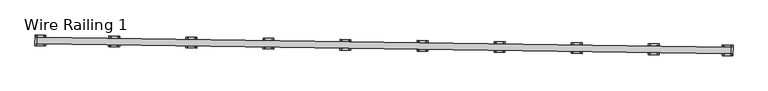
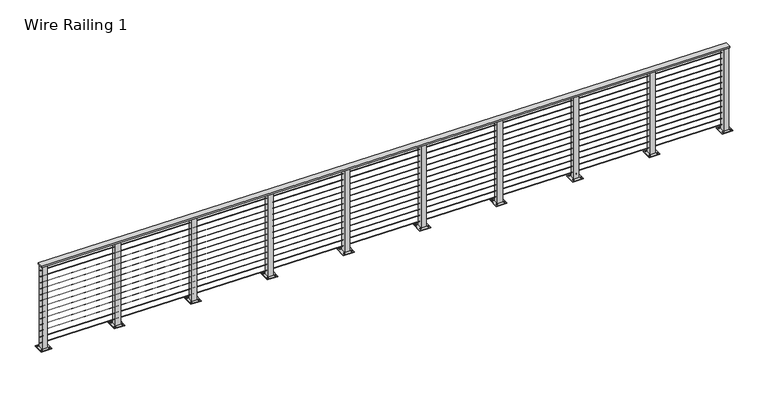
"""IFC4 building model written with IfcOpenShell, lengths in millimetres: railing geometry, Wire Railing 1."""

import ifcopenshell
import ifcopenshell.guid

model = None  # the IFC model being written
_history = None  # IfcOwnerHistory: only IFC2X3 demands one
_inside = {}  # id of a spatial element -> (the spatial element, [elements in it])
_under = {}  # id of a project, library or spatial element -> (it, [spatial elements below it])
_declared = {}  # id of a project -> (the project, [libraries it declares])
_typed = {}  # id of a type object -> (the type object, [elements of that type])
_made_of = {}  # id of a material, layer set ... -> (it, [elements and type objects made of it])


def new_model(schema):
    """Start an empty IFC model of exactly this schema.

    Asked for "IFC4X3", IfcOpenShell would pick the latest addendum, in which some entities
    have other attributes; the version numbers below select the first issue.
    IFC2X3 requires an IfcOwnerHistory on every rooted entity: one is made here for all.
    """
    global model, _history
    if schema == "IFC4X3":
        model = ifcopenshell.file(schema_version=(4, 3, 0, 0))
    else:
        model = ifcopenshell.file(schema=schema)
    _inside.clear()
    _under.clear()
    _declared.clear()
    _typed.clear()
    _made_of.clear()
    _history = None
    if model.schema == "IFC2X3":
        org = make("IfcOrganization", Name="unknown")
        user = make(
            "IfcPersonAndOrganization",
            ThePerson=make("IfcPerson", FamilyName="unknown"),
            TheOrganization=org,
        )
        app = make(
            "IfcApplication",
            ApplicationDeveloper=org,
            Version="unknown",
            ApplicationFullName="unknown",
            ApplicationIdentifier="unknown",
        )
        _history = make(
            "IfcOwnerHistory",
            OwningUser=user,
            OwningApplication=app,
            ChangeAction="ADDED",
            CreationDate=0,
        )
    return model


def make(cls, **values):
    """One entity of the class cls with the attributes given. An attribute that is None is left unset."""
    return model.create_entity(
        cls, **{name: value for name, value in values.items() if value is not None}
    )


def rooted(cls, **values):
    """An entity with a GlobalId (a new one), such as an element, a storey or a relation."""
    return make(cls, GlobalId=ifcopenshell.guid.new(), OwnerHistory=_history, **values)


def si_unit(unit_type, name, prefix=None):
    """IfcSIUnit, for example si_unit("LENGTHUNIT", "METRE", prefix="MILLI")."""
    return make("IfcSIUnit", UnitType=unit_type, Prefix=prefix, Name=name)


def assignment(units):
    """IfcUnitAssignment: the units of a project."""
    return None if units is None else make("IfcUnitAssignment", Units=units)


def point(xyz):
    """IfcCartesianPoint."""
    return None if xyz is None else make("IfcCartesianPoint", Coordinates=xyz)


def direction(xyz):
    """IfcDirection."""
    return None if xyz is None else make("IfcDirection", DirectionRatios=xyz)


def frame(location, z_axis=None, x_axis=None):
    """IfcAxis2Placement3D, a coordinate frame: its origin and axes. An axis left out is left unset."""
    return make(
        "IfcAxis2Placement3D",
        Location=point(location),
        Axis=direction(z_axis),
        RefDirection=direction(x_axis),
    )


def frame_2d(location, x_axis=None):
    """IfcAxis2Placement2D, a coordinate frame in the plane: its origin and x axis."""
    return make(
        "IfcAxis2Placement2D", Location=point(location), RefDirection=direction(x_axis)
    )


def origin():
    """The frame at (0, 0, 0) with its axes left unset."""
    return frame((0.0, 0.0, 0.0))


def place(relative_to, where):
    """IfcLocalPlacement: puts the frame where relative to a parent placement (None: the world)."""
    return make(
        "IfcLocalPlacement", PlacementRelTo=relative_to, RelativePlacement=where
    )


def context(
    kind, dimensions, precision=None, world=None, true_north=None, identifier=None
):
    """IfcGeometricRepresentationContext, for example the 3D "Model" context."""
    return make(
        "IfcGeometricRepresentationContext",
        ContextIdentifier=identifier,
        ContextType=kind,
        CoordinateSpaceDimension=dimensions,
        Precision=precision,
        WorldCoordinateSystem=world,
        TrueNorth=true_north,
    )


def project(units=None, contexts=None):
    """IfcProject with its units and contexts."""
    return rooted(
        "IfcProject",
        Name="project",
        RepresentationContexts=contexts,
        UnitsInContext=assignment(units),
    )


def spatial(cls, under=None, at=None, **own):
    """A site, building, storey or space (cls), placed at a placement, below another one or the project."""
    s = rooted(cls, ObjectPlacement=at, **own)
    if under is not None:
        _under.setdefault(under.id(), (under, []))[1].append(s)
    return s


def polyline(points):
    """IfcPolyline through the points."""
    return make("IfcPolyline", Points=[point(p) for p in points])


def circle_curve(where, radius):
    """IfcCircle in the frame where."""
    return make("IfcCircle", Position=where, Radius=radius)


def trimmed(basis, trim1, trim2, sense, master):
    """IfcTrimmedCurve: the piece of a basis curve between two trims."""
    return make(
        "IfcTrimmedCurve",
        BasisCurve=basis,
        Trim1=trim1,
        Trim2=trim2,
        SenseAgreement=sense,
        MasterRepresentation=master,
    )


def segment(curve, same_sense, transition):
    """IfcCompositeCurveSegment."""
    return make(
        "IfcCompositeCurveSegment",
        Transition=transition,
        SameSense=same_sense,
        ParentCurve=curve,
    )


def composite_curve(segments, self_intersect=None):
    """IfcCompositeCurve: segments joined end to end."""
    return make("IfcCompositeCurve", Segments=segments, SelfIntersect=self_intersect)


def outline(outer, holes=None, kind="AREA"):
    """IfcArbitraryClosedProfileDef: a profile drawn as a closed curve; with holes, ...WithVoids."""
    if holes is None:
        return make("IfcArbitraryClosedProfileDef", ProfileType=kind, OuterCurve=outer)
    return make(
        "IfcArbitraryProfileDefWithVoids",
        ProfileType=kind,
        OuterCurve=outer,
        InnerCurves=holes,
    )


def extrude(swept, where, along, depth):
    """IfcExtrudedAreaSolid: the profile swept, set in the frame where, extruded along a direction by depth."""
    return make(
        "IfcExtrudedAreaSolid",
        SweptArea=swept,
        Position=where,
        ExtrudedDirection=direction(along),
        Depth=depth,
    )


def shape(context_of_items, identifier, shape_type, items):
    """IfcShapeRepresentation: the items that make up one representation, for example the "Body"."""
    return make(
        "IfcShapeRepresentation",
        ContextOfItems=context_of_items,
        RepresentationIdentifier=identifier,
        RepresentationType=shape_type,
        Items=items,
    )


def source(mapping_origin, context_of_items, identifier, shape_type, items):
    """IfcRepresentationMap: a shape defined once, which mapped items show again and again."""
    return make(
        "IfcRepresentationMap",
        MappingOrigin=mapping_origin,
        MappedRepresentation=shape(context_of_items, identifier, shape_type, items),
    )


def transform(
    local_origin,
    x_axis=None,
    y_axis=None,
    z_axis=None,
    scale=None,
    scale2=None,
    scale3=None,
    uniform=True,
):
    """IfcCartesianTransformationOperator3D, or its non-uniform kind. x_axis, y_axis, z_axis: its Axis1, 2, 3."""
    if uniform:
        return make(
            "IfcCartesianTransformationOperator3D",
            Axis1=direction(x_axis),
            Axis2=direction(y_axis),
            LocalOrigin=point(local_origin),
            Scale=scale,
            Axis3=direction(z_axis),
        )
    return make(
        "IfcCartesianTransformationOperator3DnonUniform",
        Axis1=direction(x_axis),
        Axis2=direction(y_axis),
        LocalOrigin=point(local_origin),
        Scale=scale,
        Axis3=direction(z_axis),
        Scale2=scale2,
        Scale3=scale3,
    )


def mapped(mapping_source, mapping_target):
    """IfcMappedItem: shows the shape of a source again, moved by a transform."""
    return make(
        "IfcMappedItem", MappingSource=mapping_source, MappingTarget=mapping_target
    )


def made_of(thing, what):
    """Note that an element or type object is made of a material, layer set ...; save() writes the relation."""
    if what is not None:
        _made_of.setdefault(what.id(), (what, []))[1].append(thing)
    return thing


def element(
    cls,
    number,
    at=None,
    inside=None,
    cuts=None,
    type_object=None,
    material=None,
    context=None,
    identifier="Body",
    shape_type=None,
    held_by="IfcProductDefinitionShape",
    body=None,
    shapes=None,
    **own,
):
    """One element of the class cls, such as IfcWall. Its Tag is "e" and its number.

    at: its placement. inside: the storey or other place that contains it. cuts: it is an
    opening in that element (IfcRelVoidsElement). A single representation is given by context,
    identifier, shape_type and body (its items); several are given by shapes. held_by: the class
    of the entity that holds the representations. save() writes the other relations.
    """
    e = rooted(cls, Tag="e%d" % number, ObjectPlacement=at, **own)
    if body is not None:
        shapes = [shape(context, identifier, shape_type, body)]
    if shapes is not None:
        e.Representation = make(held_by, Representations=shapes)
    if inside is not None:
        _inside.setdefault(inside.id(), (inside, []))[1].append(e)
    if cuts is not None:
        rooted(
            "IfcRelVoidsElement", RelatingBuildingElement=cuts, RelatedOpeningElement=e
        )
    if type_object is not None:
        _typed.setdefault(type_object.id(), (type_object, []))[1].append(e)
    return made_of(e, material)


def aggregate(whole, parts):
    """IfcRelAggregates: a whole, such as a stair, and the parts it consists of."""
    return rooted("IfcRelAggregates", RelatingObject=whole, RelatedObjects=parts)


def save(model, path):
    """Write the relations noted so far, then the file.

    IfcRelAggregates (storeys below a building ...), IfcRelContainedInSpatialStructure (elements
    in a storey), IfcRelDefinesByType, IfcRelAssociatesMaterial and IfcRelDeclares: one each for
    every whole, place, type object, material and project.
    """
    for whole, parts in _under.values():
        aggregate(whole, parts)
    for where, things in _inside.values():
        rooted(
            "IfcRelContainedInSpatialStructure",
            RelatedElements=things,
            RelatingStructure=where,
        )
    for kind, things in _typed.values():
        rooted("IfcRelDefinesByType", RelatedObjects=things, RelatingType=kind)
    for what, things in _made_of.values():
        rooted("IfcRelAssociatesMaterial", RelatedObjects=things, RelatingMaterial=what)
    for by, libraries in _declared.values():
        rooted("IfcRelDeclares", RelatingContext=by, RelatedDefinitions=libraries)
    model.write(path)


def wire_railing_1_a1e0410e(model_context):
    return source(origin(), model_context, "Body", "SweptSolid", [
        extrude(outline(polyline([(37771.61111, 41116.6903906), (37772.7149224, 41192.8823954), (45955.2738821, 41074.3396493), (45954.1700698, 40998.1476444), (37771.61111, 41116.6903906)])), frame((0.0, 0.0, 267138.15), z_axis=(0.0, 0.0, 1.0), x_axis=(1.0, 0.0, 0.0)), (0.0, 0.0, 1.0), 19.05),
        extrude(outline(composite_curve([segment(trimmed(circle_curve(frame_2d((0.0, 2.38125)), 2.38125), [point((2.3812499, 2.38125))], [point((-2.3812501, 2.38125))], False, "CARTESIAN"), True, "CONTINUOUS"), segment(trimmed(circle_curve(frame_2d((0.0, 2.38125)), 2.38125), [point((-2.3812501, 2.38125))], [point((2.3812499, 2.38125))], False, "CARTESIAN"), True, "CONTINUOUS")], self_intersect=False)), frame((45954.721976, 41036.2436469, 267081.0), z_axis=(-0.9998950763646337, 0.014485726138629394, 0.0), x_axis=(0.014485726138629394, 0.9998950763646337, 0.0)), (0.0, 0.0, 1.0), 8183.4175937),
        extrude(outline(composite_curve([segment(trimmed(circle_curve(frame_2d((0.0, 2.38125)), 2.38125), [point((2.3812499, 2.38125))], [point((-2.3812501, 2.38125))], False, "CARTESIAN"), True, "CONTINUOUS"), segment(trimmed(circle_curve(frame_2d((0.0, 2.38125)), 2.38125), [point((-2.3812501, 2.38125))], [point((2.3812499, 2.38125))], False, "CARTESIAN"), True, "CONTINUOUS")], self_intersect=False)), frame((45954.721976, 41036.2436469, 267004.8), z_axis=(-0.9998950763646337, 0.014485726138629394, 0.0), x_axis=(0.014485726138629394, 0.9998950763646337, 0.0)), (0.0, 0.0, 1.0), 8183.4175937),
        extrude(outline(composite_curve([segment(trimmed(circle_curve(frame_2d((0.0, 2.38125)), 2.38125), [point((2.3812499, 2.38125))], [point((-2.3812501, 2.38125))], False, "CARTESIAN"), True, "CONTINUOUS"), segment(trimmed(circle_curve(frame_2d((0.0, 2.38125)), 2.38125), [point((-2.3812501, 2.38125))], [point((2.3812499, 2.38125))], False, "CARTESIAN"), True, "CONTINUOUS")], self_intersect=False)), frame((45954.721976, 41036.2436469, 266928.6), z_axis=(-0.9998950763646337, 0.014485726138629394, 0.0), x_axis=(0.014485726138629394, 0.9998950763646337, 0.0)), (0.0, 0.0, 1.0), 8183.4175937),
        extrude(outline(composite_curve([segment(trimmed(circle_curve(frame_2d((0.0, 2.38125)), 2.38125), [point((2.3812499, 2.38125))], [point((-2.3812501, 2.38125))], False, "CARTESIAN"), True, "CONTINUOUS"), segment(trimmed(circle_curve(frame_2d((0.0, 2.38125)), 2.38125), [point((-2.3812501, 2.38125))], [point((2.3812499, 2.38125))], False, "CARTESIAN"), True, "CONTINUOUS")], self_intersect=False)), frame((45954.721976, 41036.2436469, 266852.4), z_axis=(-0.9998950763646337, 0.014485726138629394, 0.0), x_axis=(0.014485726138629394, 0.9998950763646337, 0.0)), (0.0, 0.0, 1.0), 8183.4175937),
        extrude(outline(composite_curve([segment(trimmed(circle_curve(frame_2d((0.0, 2.38125)), 2.38125), [point((2.3812499, 2.38125))], [point((-2.3812501, 2.38125))], False, "CARTESIAN"), True, "CONTINUOUS"), segment(trimmed(circle_curve(frame_2d((0.0, 2.38125)), 2.38125), [point((-2.3812501, 2.38125))], [point((2.3812499, 2.38125))], False, "CARTESIAN"), True, "CONTINUOUS")], self_intersect=False)), frame((45954.721976, 41036.2436469, 266776.2), z_axis=(-0.9998950763646337, 0.014485726138629394, 0.0), x_axis=(0.014485726138629394, 0.9998950763646337, 0.0)), (0.0, 0.0, 1.0), 8183.4175937),
        extrude(outline(composite_curve([segment(trimmed(circle_curve(frame_2d((0.0, 2.38125)), 2.38125), [point((2.3812499, 2.38125))], [point((-2.3812501, 2.38125))], False, "CARTESIAN"), True, "CONTINUOUS"), segment(trimmed(circle_curve(frame_2d((0.0, 2.38125)), 2.38125), [point((-2.3812501, 2.38125))], [point((2.3812499, 2.38125))], False, "CARTESIAN"), True, "CONTINUOUS")], self_intersect=False)), frame((45954.721976, 41036.2436469, 266700.0), z_axis=(-0.9998950763646337, 0.014485726138629394, 0.0), x_axis=(0.014485726138629394, 0.9998950763646337, 0.0)), (0.0, 0.0, 1.0), 8183.4175937),
        extrude(outline(composite_curve([segment(trimmed(circle_curve(frame_2d((0.0, 2.38125)), 2.38125), [point((2.3812499, 2.38125))], [point((-2.3812501, 2.38125))], False, "CARTESIAN"), True, "CONTINUOUS"), segment(trimmed(circle_curve(frame_2d((0.0, 2.38125)), 2.38125), [point((-2.3812501, 2.38125))], [point((2.3812499, 2.38125))], False, "CARTESIAN"), True, "CONTINUOUS")], self_intersect=False)), frame((45954.721976, 41036.2436469, 266623.8), z_axis=(-0.9998950763646337, 0.014485726138629394, 0.0), x_axis=(0.014485726138629394, 0.9998950763646337, 0.0)), (0.0, 0.0, 1.0), 8183.4175937),
        extrude(outline(composite_curve([segment(trimmed(circle_curve(frame_2d((0.0, 2.38125)), 2.38125), [point((2.3812499, 2.38125))], [point((-2.3812501, 2.38125))], False, "CARTESIAN"), True, "CONTINUOUS"), segment(trimmed(circle_curve(frame_2d((0.0, 2.38125)), 2.38125), [point((-2.3812501, 2.38125))], [point((2.3812499, 2.38125))], False, "CARTESIAN"), True, "CONTINUOUS")], self_intersect=False)), frame((45954.721976, 41036.2436469, 266547.6), z_axis=(-0.9998950763646337, 0.014485726138629394, 0.0), x_axis=(0.014485726138629394, 0.9998950763646337, 0.0)), (0.0, 0.0, 1.0), 8183.4175937),
        extrude(outline(composite_curve([segment(trimmed(circle_curve(frame_2d((0.0, 2.38125)), 2.38125), [point((2.3812499, 2.38125))], [point((-2.3812501, 2.38125))], False, "CARTESIAN"), True, "CONTINUOUS"), segment(trimmed(circle_curve(frame_2d((0.0, 2.38125)), 2.38125), [point((-2.3812501, 2.38125))], [point((2.3812499, 2.38125))], False, "CARTESIAN"), True, "CONTINUOUS")], self_intersect=False)), frame((45954.721976, 41036.2436469, 266471.4), z_axis=(-0.9998950763646337, 0.014485726138629394, 0.0), x_axis=(0.014485726138629394, 0.9998950763646337, 0.0)), (0.0, 0.0, 1.0), 8183.4175937),
        extrude(outline(composite_curve([segment(trimmed(circle_curve(frame_2d((0.0, 2.38125)), 2.38125), [point((2.3812499, 2.38125))], [point((-2.3812501, 2.38125))], False, "CARTESIAN"), True, "CONTINUOUS"), segment(trimmed(circle_curve(frame_2d((0.0, 2.38125)), 2.38125), [point((-2.3812501, 2.38125))], [point((2.3812499, 2.38125))], False, "CARTESIAN"), True, "CONTINUOUS")], self_intersect=False)), frame((45954.721976, 41036.2436469, 266395.2), z_axis=(-0.9998950763646337, 0.014485726138629394, 0.0), x_axis=(0.014485726138629394, 0.9998950763646337, 0.0)), (0.0, 0.0, 1.0), 8183.4175937),
        extrude(outline(composite_curve([segment(trimmed(circle_curve(frame_2d((0.0, 2.38125)), 2.38125), [point((2.3812499, 2.38125))], [point((-2.3812501, 2.38125))], False, "CARTESIAN"), True, "CONTINUOUS"), segment(trimmed(circle_curve(frame_2d((0.0, 2.38125)), 2.38125), [point((-2.3812501, 2.38125))], [point((2.3812499, 2.38125))], False, "CARTESIAN"), True, "CONTINUOUS")], self_intersect=False)), frame((45954.721976, 41036.2436469, 266319.0), z_axis=(-0.9998950763646337, 0.014485726138629394, 0.0), x_axis=(0.014485726138629394, 0.9998950763646337, 0.0)), (0.0, 0.0, 1.0), 8183.4175937),
        extrude(outline(composite_curve([segment(trimmed(circle_curve(frame_2d((0.0, 2.38125)), 2.38125), [point((2.3812499, 2.38125))], [point((-2.3812501, 2.38125))], False, "CARTESIAN"), True, "CONTINUOUS"), segment(trimmed(circle_curve(frame_2d((0.0, 2.38125)), 2.38125), [point((-2.3812501, 2.38125))], [point((2.3812499, 2.38125))], False, "CARTESIAN"), True, "CONTINUOUS")], self_intersect=False)), frame((45954.721976, 41036.2436469, 266242.8), z_axis=(-0.9998950763646337, 0.014485726138629394, 0.0), x_axis=(0.014485726138629394, 0.9998950763646337, 0.0)), (0.0, 0.0, 1.0), 8183.4175937),
        extrude(outline(composite_curve([segment(trimmed(circle_curve(frame_2d((0.0, 2.38125)), 2.38125), [point((2.3812499, 2.38125))], [point((-2.3812501, 2.38125))], False, "CARTESIAN"), True, "CONTINUOUS"), segment(trimmed(circle_curve(frame_2d((0.0, 2.38125)), 2.38125), [point((-2.3812501, 2.38125))], [point((2.3812499, 2.38125))], False, "CARTESIAN"), True, "CONTINUOUS")], self_intersect=False)), frame((45954.721976, 41036.2436469, 266166.6), z_axis=(-0.9998950763646337, 0.014485726138629394, 0.0), x_axis=(0.014485726138629394, 0.9998950763646337, 0.0)), (0.0, 0.0, 1.0), 8183.4175937),
        extrude(outline(composite_curve([segment(trimmed(circle_curve(frame_2d((45000.4595315, 41005.6136175)), 6.35), [point((45000.3675472, 40999.2642837))], [point((45000.5515159, 41011.9629512))], False, "CARTESIAN"), True, "CONTINUOUS"), segment(trimmed(circle_curve(frame_2d((45000.4595315, 41005.6136175)), 6.35), [point((45000.5515159, 41011.9629512))], [point((45000.3675472, 40999.2642837))], False, "CARTESIAN"), True, "CONTINUOUS")], self_intersect=False)), frame((0.0, 0.0, 266090.4), z_axis=(0.0, 0.0, 1.0), x_axis=(1.0, 0.0, 0.0)), (0.0, 0.0, 1.0), 12.7),
        extrude(outline(composite_curve([segment(trimmed(circle_curve(frame_2d((45001.7473126, 41094.5042898)), 6.35), [point((45001.6553282, 41088.154956))], [point((45001.8392969, 41100.8536235))], False, "CARTESIAN"), True, "CONTINUOUS"), segment(trimmed(circle_curve(frame_2d((45001.7473126, 41094.5042898)), 6.35), [point((45001.8392969, 41100.8536235))], [point((45001.6553282, 41088.154956))], False, "CARTESIAN"), True, "CONTINUOUS")], self_intersect=False)), frame((0.0, 0.0, 266090.4), z_axis=(0.0, 0.0, 1.0), x_axis=(1.0, 0.0, 0.0)), (0.0, 0.0, 1.0), 12.7),
        extrude(outline(composite_curve([segment(trimmed(circle_curve(frame_2d((45089.3502038, 41004.3258364)), 6.35), [point((45089.2582195, 40997.9765027))], [point((45089.4421882, 41010.6751702))], False, "CARTESIAN"), True, "CONTINUOUS"), segment(trimmed(circle_curve(frame_2d((45089.3502038, 41004.3258364)), 6.35), [point((45089.4421882, 41010.6751702))], [point((45089.2582195, 40997.9765027))], False, "CARTESIAN"), True, "CONTINUOUS")], self_intersect=False)), frame((0.0, 0.0, 266090.4), z_axis=(0.0, 0.0, 1.0), x_axis=(1.0, 0.0, 0.0)), (0.0, 0.0, 1.0), 12.7),
        extrude(outline(composite_curve([segment(trimmed(circle_curve(frame_2d((45090.6379849, 41093.2165087)), 6.35), [point((45090.5460005, 41086.867175))], [point((45090.7299692, 41099.5658424))], False, "CARTESIAN"), True, "CONTINUOUS"), segment(trimmed(circle_curve(frame_2d((45090.6379849, 41093.2165087)), 6.35), [point((45090.7299692, 41099.5658424))], [point((45090.5460005, 41086.867175))], False, "CARTESIAN"), True, "CONTINUOUS")], self_intersect=False)), frame((0.0, 0.0, 266090.4), z_axis=(0.0, 0.0, 1.0), x_axis=(1.0, 0.0, 0.0)), (0.0, 0.0, 1.0), 12.7),
        extrude(outline(polyline([(44982.9752645, 41113.8282441), (45109.9619392, 41111.9885568), (45108.1222519, 40985.0018821), (44981.1355772, 40986.8415694), (44982.9752645, 41113.8282441)])), frame((0.0, 0.0, 266090.4), z_axis=(0.0, 0.0, 1.0), x_axis=(1.0, 0.0, 0.0)), (0.0, 0.0, 1.0), 6.35),
        extrude(outline(polyline([(45015.8263487, 41080.011324), (45076.1450192, 41079.1374726), (45075.2711677, 41018.8188021), (45014.9524972, 41019.6926536), (45015.8263487, 41080.011324)]), holes=[polyline([(45022.0836981, 41073.570006), (45021.3938153, 41025.9500029), (45069.0138184, 41025.2601202), (45069.7037011, 41072.8801232), (45022.0836981, 41073.570006)])]), frame((0.0, 0.0, 266090.4), z_axis=(0.0, 0.0, 1.0), x_axis=(1.0, 0.0, 0.0)), (0.0, 0.0, 1.0), 1047.75),
        extrude(outline(composite_curve([segment(trimmed(circle_curve(frame_2d((44091.2863138, 41018.7850337)), 6.35), [point((44091.1943294, 41012.4357))], [point((44091.3782981, 41025.1343674))], False, "CARTESIAN"), True, "CONTINUOUS"), segment(trimmed(circle_curve(frame_2d((44091.2863138, 41018.7850337)), 6.35), [point((44091.3782981, 41025.1343674))], [point((44091.1943294, 41012.4357))], False, "CARTESIAN"), True, "CONTINUOUS")], self_intersect=False)), frame((0.0, 0.0, 266090.4), z_axis=(0.0, 0.0, 1.0), x_axis=(1.0, 0.0, 0.0)), (0.0, 0.0, 1.0), 12.7),
        extrude(outline(composite_curve([segment(trimmed(circle_curve(frame_2d((44092.5740948, 41107.675706)), 6.35), [point((44092.4821105, 41101.3263723))], [point((44092.6660792, 41114.0250397))], False, "CARTESIAN"), True, "CONTINUOUS"), segment(trimmed(circle_curve(frame_2d((44092.5740948, 41107.675706)), 6.35), [point((44092.6660792, 41114.0250397))], [point((44092.4821105, 41101.3263723))], False, "CARTESIAN"), True, "CONTINUOUS")], self_intersect=False)), frame((0.0, 0.0, 266090.4), z_axis=(0.0, 0.0, 1.0), x_axis=(1.0, 0.0, 0.0)), (0.0, 0.0, 1.0), 12.7),
        extrude(outline(composite_curve([segment(trimmed(circle_curve(frame_2d((44180.1769861, 41017.4972527)), 6.35), [point((44180.0850017, 41011.1479189))], [point((44180.2689704, 41023.8465864))], False, "CARTESIAN"), True, "CONTINUOUS"), segment(trimmed(circle_curve(frame_2d((44180.1769861, 41017.4972527)), 6.35), [point((44180.2689704, 41023.8465864))], [point((44180.0850017, 41011.1479189))], False, "CARTESIAN"), True, "CONTINUOUS")], self_intersect=False)), frame((0.0, 0.0, 266090.4), z_axis=(0.0, 0.0, 1.0), x_axis=(1.0, 0.0, 0.0)), (0.0, 0.0, 1.0), 12.7),
        extrude(outline(composite_curve([segment(trimmed(circle_curve(frame_2d((44181.4647671, 41106.3879249)), 6.35), [point((44181.3727828, 41100.0385912))], [point((44181.5567515, 41112.7372587))], False, "CARTESIAN"), True, "CONTINUOUS"), segment(trimmed(circle_curve(frame_2d((44181.4647671, 41106.3879249)), 6.35), [point((44181.5567515, 41112.7372587))], [point((44181.3727828, 41100.0385912))], False, "CARTESIAN"), True, "CONTINUOUS")], self_intersect=False)), frame((0.0, 0.0, 266090.4), z_axis=(0.0, 0.0, 1.0), x_axis=(1.0, 0.0, 0.0)), (0.0, 0.0, 1.0), 12.7),
        extrude(outline(polyline([(44073.8020467, 41126.9996603), (44200.7887214, 41125.1599731), (44198.9490342, 40998.1732984), (44071.9623595, 41000.0129856), (44073.8020467, 41126.9996603)])), frame((0.0, 0.0, 266090.4), z_axis=(0.0, 0.0, 1.0), x_axis=(1.0, 0.0, 0.0)), (0.0, 0.0, 1.0), 6.35),
        extrude(outline(polyline([(44106.6531309, 41093.1827403), (44166.9718014, 41092.3088889), (44166.09795, 41031.9902184), (44105.7792795, 41032.8640698), (44106.6531309, 41093.1827403)]), holes=[polyline([(44112.9104803, 41086.7414222), (44112.2205976, 41039.1214192), (44159.8406006, 41038.4315365), (44160.5304833, 41086.0515395), (44112.9104803, 41086.7414222)])]), frame((0.0, 0.0, 266090.4), z_axis=(0.0, 0.0, 1.0), x_axis=(1.0, 0.0, 0.0)), (0.0, 0.0, 1.0), 1047.75),
        extrude(outline(composite_curve([segment(trimmed(circle_curve(frame_2d((43182.113096, 41031.95645)), 6.35), [point((43182.0211117, 41025.6071162))], [point((43182.2050804, 41038.3057837))], False, "CARTESIAN"), True, "CONTINUOUS"), segment(trimmed(circle_curve(frame_2d((43182.113096, 41031.95645)), 6.35), [point((43182.2050804, 41038.3057837))], [point((43182.0211117, 41025.6071162))], False, "CARTESIAN"), True, "CONTINUOUS")], self_intersect=False)), frame((0.0, 0.0, 266090.4), z_axis=(0.0, 0.0, 1.0), x_axis=(1.0, 0.0, 0.0)), (0.0, 0.0, 1.0), 12.7),
        extrude(outline(composite_curve([segment(trimmed(circle_curve(frame_2d((43183.4008771, 41120.8471222)), 6.35), [point((43183.3088927, 41114.4977885))], [point((43183.4928614, 41127.196456))], False, "CARTESIAN"), True, "CONTINUOUS"), segment(trimmed(circle_curve(frame_2d((43183.4008771, 41120.8471222)), 6.35), [point((43183.4928614, 41127.196456))], [point((43183.3088927, 41114.4977885))], False, "CARTESIAN"), True, "CONTINUOUS")], self_intersect=False)), frame((0.0, 0.0, 266090.4), z_axis=(0.0, 0.0, 1.0), x_axis=(1.0, 0.0, 0.0)), (0.0, 0.0, 1.0), 12.7),
        extrude(outline(composite_curve([segment(trimmed(circle_curve(frame_2d((43271.0037683, 41030.6686689)), 6.35), [point((43270.911784, 41024.3193352))], [point((43271.0957527, 41037.0180026))], False, "CARTESIAN"), True, "CONTINUOUS"), segment(trimmed(circle_curve(frame_2d((43271.0037683, 41030.6686689)), 6.35), [point((43271.0957527, 41037.0180026))], [point((43270.911784, 41024.3193352))], False, "CARTESIAN"), True, "CONTINUOUS")], self_intersect=False)), frame((0.0, 0.0, 266090.4), z_axis=(0.0, 0.0, 1.0), x_axis=(1.0, 0.0, 0.0)), (0.0, 0.0, 1.0), 12.7),
        extrude(outline(composite_curve([segment(trimmed(circle_curve(frame_2d((43272.2915494, 41119.5593412)), 6.35), [point((43272.199565, 41113.2100075))], [point((43272.3835337, 41125.9086749))], False, "CARTESIAN"), True, "CONTINUOUS"), segment(trimmed(circle_curve(frame_2d((43272.2915494, 41119.5593412)), 6.35), [point((43272.3835337, 41125.9086749))], [point((43272.199565, 41113.2100075))], False, "CARTESIAN"), True, "CONTINUOUS")], self_intersect=False)), frame((0.0, 0.0, 266090.4), z_axis=(0.0, 0.0, 1.0), x_axis=(1.0, 0.0, 0.0)), (0.0, 0.0, 1.0), 12.7),
        extrude(outline(polyline([(43164.628829, 41140.1710765), (43291.6155037, 41138.3313893), (43289.7758164, 41011.3447146), (43162.7891417, 41013.1844018), (43164.628829, 41140.1710765)])), frame((0.0, 0.0, 266090.4), z_axis=(0.0, 0.0, 1.0), x_axis=(1.0, 0.0, 0.0)), (0.0, 0.0, 1.0), 6.35),
        extrude(outline(polyline([(43197.4799132, 41106.3541565), (43257.7985837, 41105.4803051), (43256.9247322, 41045.1616346), (43196.6060618, 41046.035486), (43197.4799132, 41106.3541565)]), holes=[polyline([(43203.7372626, 41099.9128384), (43203.0473798, 41052.2928354), (43250.6673829, 41051.6029527), (43251.3572656, 41099.2229557), (43203.7372626, 41099.9128384)])]), frame((0.0, 0.0, 266090.4), z_axis=(0.0, 0.0, 1.0), x_axis=(1.0, 0.0, 0.0)), (0.0, 0.0, 1.0), 1047.75),
        extrude(outline(composite_curve([segment(trimmed(circle_curve(frame_2d((42272.9398783, 41045.1278662)), 6.35), [point((42272.8478939, 41038.7785325))], [point((42273.0318626, 41051.4771999))], False, "CARTESIAN"), True, "CONTINUOUS"), segment(trimmed(circle_curve(frame_2d((42272.9398783, 41045.1278662)), 6.35), [point((42273.0318626, 41051.4771999))], [point((42272.8478939, 41038.7785325))], False, "CARTESIAN"), True, "CONTINUOUS")], self_intersect=False)), frame((0.0, 0.0, 266090.4), z_axis=(0.0, 0.0, 1.0), x_axis=(1.0, 0.0, 0.0)), (0.0, 0.0, 1.0), 12.7),
        extrude(outline(composite_curve([segment(trimmed(circle_curve(frame_2d((42274.2276593, 41134.0185385)), 6.35), [point((42274.135675, 41127.6692047))], [point((42274.3196437, 41140.3678722))], False, "CARTESIAN"), True, "CONTINUOUS"), segment(trimmed(circle_curve(frame_2d((42274.2276593, 41134.0185385)), 6.35), [point((42274.3196437, 41140.3678722))], [point((42274.135675, 41127.6692047))], False, "CARTESIAN"), True, "CONTINUOUS")], self_intersect=False)), frame((0.0, 0.0, 266090.4), z_axis=(0.0, 0.0, 1.0), x_axis=(1.0, 0.0, 0.0)), (0.0, 0.0, 1.0), 12.7),
        extrude(outline(composite_curve([segment(trimmed(circle_curve(frame_2d((42361.8305506, 41043.8400851)), 6.35), [point((42361.7385662, 41037.4907514))], [point((42361.9225349, 41050.1894189))], False, "CARTESIAN"), True, "CONTINUOUS"), segment(trimmed(circle_curve(frame_2d((42361.8305506, 41043.8400851)), 6.35), [point((42361.9225349, 41050.1894189))], [point((42361.7385662, 41037.4907514))], False, "CARTESIAN"), True, "CONTINUOUS")], self_intersect=False)), frame((0.0, 0.0, 266090.4), z_axis=(0.0, 0.0, 1.0), x_axis=(1.0, 0.0, 0.0)), (0.0, 0.0, 1.0), 12.7),
        extrude(outline(composite_curve([segment(trimmed(circle_curve(frame_2d((42363.1183316, 41132.7307574)), 6.35), [point((42363.0263473, 41126.3814237))], [point((42363.210316, 41139.0800912))], False, "CARTESIAN"), True, "CONTINUOUS"), segment(trimmed(circle_curve(frame_2d((42363.1183316, 41132.7307574)), 6.35), [point((42363.210316, 41139.0800912))], [point((42363.0263473, 41126.3814237))], False, "CARTESIAN"), True, "CONTINUOUS")], self_intersect=False)), frame((0.0, 0.0, 266090.4), z_axis=(0.0, 0.0, 1.0), x_axis=(1.0, 0.0, 0.0)), (0.0, 0.0, 1.0), 12.7),
        extrude(outline(polyline([(42255.4556112, 41153.3424928), (42382.4422859, 41151.5028055), (42380.6025987, 41024.5161308), (42253.615924, 41026.3558181), (42255.4556112, 41153.3424928)])), frame((0.0, 0.0, 266090.4), z_axis=(0.0, 0.0, 1.0), x_axis=(1.0, 0.0, 0.0)), (0.0, 0.0, 1.0), 6.35),
        extrude(outline(polyline([(42288.3066954, 41119.5255728), (42348.6253659, 41118.6517213), (42347.7515145, 41058.3330509), (42287.432844, 41059.2069023), (42288.3066954, 41119.5255728)]), holes=[polyline([(42294.5640448, 41113.0842547), (42293.8741621, 41065.4642517), (42341.4941651, 41064.7743689), (42342.1840478, 41112.394372), (42294.5640448, 41113.0842547)])]), frame((0.0, 0.0, 266090.4), z_axis=(0.0, 0.0, 1.0), x_axis=(1.0, 0.0, 0.0)), (0.0, 0.0, 1.0), 1047.75),
        extrude(outline(composite_curve([segment(trimmed(circle_curve(frame_2d((41363.7666605, 41058.2992824)), 6.35), [point((41363.6746762, 41051.9499487))], [point((41363.8586449, 41064.6486162))], False, "CARTESIAN"), True, "CONTINUOUS"), segment(trimmed(circle_curve(frame_2d((41363.7666605, 41058.2992824)), 6.35), [point((41363.8586449, 41064.6486162))], [point((41363.6746762, 41051.9499487))], False, "CARTESIAN"), True, "CONTINUOUS")], self_intersect=False)), frame((0.0, 0.0, 266090.4), z_axis=(0.0, 0.0, 1.0), x_axis=(1.0, 0.0, 0.0)), (0.0, 0.0, 1.0), 12.7),
        extrude(outline(composite_curve([segment(trimmed(circle_curve(frame_2d((41365.0544416, 41147.1899547)), 6.35), [point((41364.9624572, 41140.840621))], [point((41365.146426, 41153.5392885))], False, "CARTESIAN"), True, "CONTINUOUS"), segment(trimmed(circle_curve(frame_2d((41365.0544416, 41147.1899547)), 6.35), [point((41365.146426, 41153.5392885))], [point((41364.9624572, 41140.840621))], False, "CARTESIAN"), True, "CONTINUOUS")], self_intersect=False)), frame((0.0, 0.0, 266090.4), z_axis=(0.0, 0.0, 1.0), x_axis=(1.0, 0.0, 0.0)), (0.0, 0.0, 1.0), 12.7),
        extrude(outline(composite_curve([segment(trimmed(circle_curve(frame_2d((41452.6573328, 41057.0115014)), 6.35), [point((41452.5653485, 41050.6621676))], [point((41452.7493172, 41063.3608351))], False, "CARTESIAN"), True, "CONTINUOUS"), segment(trimmed(circle_curve(frame_2d((41452.6573328, 41057.0115014)), 6.35), [point((41452.7493172, 41063.3608351))], [point((41452.5653485, 41050.6621676))], False, "CARTESIAN"), True, "CONTINUOUS")], self_intersect=False)), frame((0.0, 0.0, 266090.4), z_axis=(0.0, 0.0, 1.0), x_axis=(1.0, 0.0, 0.0)), (0.0, 0.0, 1.0), 12.7),
        extrude(outline(composite_curve([segment(trimmed(circle_curve(frame_2d((41453.9451139, 41145.9021737)), 6.35), [point((41453.8531295, 41139.5528399))], [point((41454.0370982, 41152.2515074))], False, "CARTESIAN"), True, "CONTINUOUS"), segment(trimmed(circle_curve(frame_2d((41453.9451139, 41145.9021737)), 6.35), [point((41454.0370982, 41152.2515074))], [point((41453.8531295, 41139.5528399))], False, "CARTESIAN"), True, "CONTINUOUS")], self_intersect=False)), frame((0.0, 0.0, 266090.4), z_axis=(0.0, 0.0, 1.0), x_axis=(1.0, 0.0, 0.0)), (0.0, 0.0, 1.0), 12.7),
        extrude(outline(polyline([(41346.2823935, 41166.513909), (41473.2690682, 41164.6742218), (41471.4293809, 41037.6875471), (41344.4427062, 41039.5272343), (41346.2823935, 41166.513909)])), frame((0.0, 0.0, 266090.4), z_axis=(0.0, 0.0, 1.0), x_axis=(1.0, 0.0, 0.0)), (0.0, 0.0, 1.0), 6.35),
        extrude(outline(polyline([(41379.1334777, 41132.696989), (41439.4521482, 41131.8231376), (41438.5782967, 41071.5044671), (41378.2596263, 41072.3783185), (41379.1334777, 41132.696989)]), holes=[polyline([(41385.3908271, 41126.2556709), (41384.7009443, 41078.6356679), (41432.3209474, 41077.9457852), (41433.0108301, 41125.5657882), (41385.3908271, 41126.2556709)])]), frame((0.0, 0.0, 266090.4), z_axis=(0.0, 0.0, 1.0), x_axis=(1.0, 0.0, 0.0)), (0.0, 0.0, 1.0), 1047.75),
        extrude(outline(composite_curve([segment(trimmed(circle_curve(frame_2d((40454.5934428, 41071.4706987)), 6.35), [point((40454.5014584, 41065.1213649))], [point((40454.6854271, 41077.8200324))], False, "CARTESIAN"), True, "CONTINUOUS"), segment(trimmed(circle_curve(frame_2d((40454.5934428, 41071.4706987)), 6.35), [point((40454.6854271, 41077.8200324))], [point((40454.5014584, 41065.1213649))], False, "CARTESIAN"), True, "CONTINUOUS")], self_intersect=False)), frame((0.0, 0.0, 266090.4), z_axis=(0.0, 0.0, 1.0), x_axis=(1.0, 0.0, 0.0)), (0.0, 0.0, 1.0), 12.7),
        extrude(outline(composite_curve([segment(trimmed(circle_curve(frame_2d((40455.8812238, 41160.361371)), 6.35), [point((40455.7892395, 41154.0120372))], [point((40455.9732082, 41166.7107047))], False, "CARTESIAN"), True, "CONTINUOUS"), segment(trimmed(circle_curve(frame_2d((40455.8812238, 41160.361371)), 6.35), [point((40455.9732082, 41166.7107047))], [point((40455.7892395, 41154.0120372))], False, "CARTESIAN"), True, "CONTINUOUS")], self_intersect=False)), frame((0.0, 0.0, 266090.4), z_axis=(0.0, 0.0, 1.0), x_axis=(1.0, 0.0, 0.0)), (0.0, 0.0, 1.0), 12.7),
        extrude(outline(composite_curve([segment(trimmed(circle_curve(frame_2d((40543.4841151, 41070.1829176)), 6.35), [point((40543.3921307, 41063.8335839))], [point((40543.5760994, 41076.5322513))], False, "CARTESIAN"), True, "CONTINUOUS"), segment(trimmed(circle_curve(frame_2d((40543.4841151, 41070.1829176)), 6.35), [point((40543.5760994, 41076.5322513))], [point((40543.3921307, 41063.8335839))], False, "CARTESIAN"), True, "CONTINUOUS")], self_intersect=False)), frame((0.0, 0.0, 266090.4), z_axis=(0.0, 0.0, 1.0), x_axis=(1.0, 0.0, 0.0)), (0.0, 0.0, 1.0), 12.7),
        extrude(outline(composite_curve([segment(trimmed(circle_curve(frame_2d((40544.7718961, 41159.0735899)), 6.35), [point((40544.6799118, 41152.7242562))], [point((40544.8638805, 41165.4229236))], False, "CARTESIAN"), True, "CONTINUOUS"), segment(trimmed(circle_curve(frame_2d((40544.7718961, 41159.0735899)), 6.35), [point((40544.8638805, 41165.4229236))], [point((40544.6799118, 41152.7242562))], False, "CARTESIAN"), True, "CONTINUOUS")], self_intersect=False)), frame((0.0, 0.0, 266090.4), z_axis=(0.0, 0.0, 1.0), x_axis=(1.0, 0.0, 0.0)), (0.0, 0.0, 1.0), 12.7),
        extrude(outline(polyline([(40437.1091757, 41179.6853252), (40564.0958504, 41177.845638), (40562.2561632, 41050.8589633), (40435.2694885, 41052.6986505), (40437.1091757, 41179.6853252)])), frame((0.0, 0.0, 266090.4), z_axis=(0.0, 0.0, 1.0), x_axis=(1.0, 0.0, 0.0)), (0.0, 0.0, 1.0), 6.35),
        extrude(outline(polyline([(40469.9602599, 41145.8684052), (40530.2789304, 41144.9945538), (40529.405079, 41084.6758833), (40469.0864085, 41085.5497348), (40469.9602599, 41145.8684052)]), holes=[polyline([(40476.2176093, 41139.4270871), (40475.5277266, 41091.8070841), (40523.1477296, 41091.1172014), (40523.8376123, 41138.7372044), (40476.2176093, 41139.4270871)])]), frame((0.0, 0.0, 266090.4), z_axis=(0.0, 0.0, 1.0), x_axis=(1.0, 0.0, 0.0)), (0.0, 0.0, 1.0), 1047.75),
        extrude(outline(composite_curve([segment(trimmed(circle_curve(frame_2d((39545.420225, 41084.6421149)), 6.35), [point((39545.3282407, 41078.2927812))], [point((39545.5122094, 41090.9914486))], False, "CARTESIAN"), True, "CONTINUOUS"), segment(trimmed(circle_curve(frame_2d((39545.420225, 41084.6421149)), 6.35), [point((39545.5122094, 41090.9914486))], [point((39545.3282407, 41078.2927812))], False, "CARTESIAN"), True, "CONTINUOUS")], self_intersect=False)), frame((0.0, 0.0, 266090.4), z_axis=(0.0, 0.0, 1.0), x_axis=(1.0, 0.0, 0.0)), (0.0, 0.0, 1.0), 12.7),
        extrude(outline(composite_curve([segment(trimmed(circle_curve(frame_2d((39546.7080061, 41173.5327872)), 6.35), [point((39546.6160217, 41167.1834535))], [point((39546.7999905, 41179.8821209))], False, "CARTESIAN"), True, "CONTINUOUS"), segment(trimmed(circle_curve(frame_2d((39546.7080061, 41173.5327872)), 6.35), [point((39546.7999905, 41179.8821209))], [point((39546.6160217, 41167.1834535))], False, "CARTESIAN"), True, "CONTINUOUS")], self_intersect=False)), frame((0.0, 0.0, 266090.4), z_axis=(0.0, 0.0, 1.0), x_axis=(1.0, 0.0, 0.0)), (0.0, 0.0, 1.0), 12.7),
        extrude(outline(composite_curve([segment(trimmed(circle_curve(frame_2d((39634.3108973, 41083.3543338)), 6.35), [point((39634.218913, 41077.0050001))], [point((39634.4028817, 41089.7036676))], False, "CARTESIAN"), True, "CONTINUOUS"), segment(trimmed(circle_curve(frame_2d((39634.3108973, 41083.3543338)), 6.35), [point((39634.4028817, 41089.7036676))], [point((39634.218913, 41077.0050001))], False, "CARTESIAN"), True, "CONTINUOUS")], self_intersect=False)), frame((0.0, 0.0, 266090.4), z_axis=(0.0, 0.0, 1.0), x_axis=(1.0, 0.0, 0.0)), (0.0, 0.0, 1.0), 12.7),
        extrude(outline(composite_curve([segment(trimmed(circle_curve(frame_2d((39635.5986784, 41172.2450061)), 6.35), [point((39635.506694, 41165.8956724))], [point((39635.6906627, 41178.5943399))], False, "CARTESIAN"), True, "CONTINUOUS"), segment(trimmed(circle_curve(frame_2d((39635.5986784, 41172.2450061)), 6.35), [point((39635.6906627, 41178.5943399))], [point((39635.506694, 41165.8956724))], False, "CARTESIAN"), True, "CONTINUOUS")], self_intersect=False)), frame((0.0, 0.0, 266090.4), z_axis=(0.0, 0.0, 1.0), x_axis=(1.0, 0.0, 0.0)), (0.0, 0.0, 1.0), 12.7),
        extrude(outline(polyline([(39527.935958, 41192.8567415), (39654.9226327, 41191.0170543), (39653.0829454, 41064.0303796), (39526.0962708, 41065.8700668), (39527.935958, 41192.8567415)])), frame((0.0, 0.0, 266090.4), z_axis=(0.0, 0.0, 1.0), x_axis=(1.0, 0.0, 0.0)), (0.0, 0.0, 1.0), 6.35),
        extrude(outline(polyline([(39560.7870422, 41159.0398215), (39621.1057127, 41158.16597), (39620.2318612, 41097.8472996), (39559.9131908, 41098.721151), (39560.7870422, 41159.0398215)]), holes=[polyline([(39567.0443916, 41152.5985034), (39566.3545089, 41104.9785004), (39613.9745119, 41104.2886177), (39614.6643946, 41151.9086207), (39567.0443916, 41152.5985034)])]), frame((0.0, 0.0, 266090.4), z_axis=(0.0, 0.0, 1.0), x_axis=(1.0, 0.0, 0.0)), (0.0, 0.0, 1.0), 1047.75),
        extrude(outline(composite_curve([segment(trimmed(circle_curve(frame_2d((38636.2470073, 41097.8135311)), 6.35), [point((38636.1550229, 41091.4641974))], [point((38636.3389917, 41104.1628649))], False, "CARTESIAN"), True, "CONTINUOUS"), segment(trimmed(circle_curve(frame_2d((38636.2470073, 41097.8135311)), 6.35), [point((38636.3389917, 41104.1628649))], [point((38636.1550229, 41091.4641974))], False, "CARTESIAN"), True, "CONTINUOUS")], self_intersect=False)), frame((0.0, 0.0, 266090.4), z_axis=(0.0, 0.0, 1.0), x_axis=(1.0, 0.0, 0.0)), (0.0, 0.0, 1.0), 12.7),
        extrude(outline(composite_curve([segment(trimmed(circle_curve(frame_2d((38637.5347883, 41186.7042034)), 6.35), [point((38637.442804, 41180.3548697))], [point((38637.6267727, 41193.0535372))], False, "CARTESIAN"), True, "CONTINUOUS"), segment(trimmed(circle_curve(frame_2d((38637.5347883, 41186.7042034)), 6.35), [point((38637.6267727, 41193.0535372))], [point((38637.442804, 41180.3548697))], False, "CARTESIAN"), True, "CONTINUOUS")], self_intersect=False)), frame((0.0, 0.0, 266090.4), z_axis=(0.0, 0.0, 1.0), x_axis=(1.0, 0.0, 0.0)), (0.0, 0.0, 1.0), 12.7),
        extrude(outline(composite_curve([segment(trimmed(circle_curve(frame_2d((38725.1376796, 41096.5257501)), 6.35), [point((38725.0456952, 41090.1764164))], [point((38725.2296639, 41102.8750838))], False, "CARTESIAN"), True, "CONTINUOUS"), segment(trimmed(circle_curve(frame_2d((38725.1376796, 41096.5257501)), 6.35), [point((38725.2296639, 41102.8750838))], [point((38725.0456952, 41090.1764164))], False, "CARTESIAN"), True, "CONTINUOUS")], self_intersect=False)), frame((0.0, 0.0, 266090.4), z_axis=(0.0, 0.0, 1.0), x_axis=(1.0, 0.0, 0.0)), (0.0, 0.0, 1.0), 12.7),
        extrude(outline(composite_curve([segment(trimmed(circle_curve(frame_2d((38726.4254606, 41185.4164224)), 6.35), [point((38726.3334763, 41179.0670886))], [point((38726.517445, 41191.7657561))], False, "CARTESIAN"), True, "CONTINUOUS"), segment(trimmed(circle_curve(frame_2d((38726.4254606, 41185.4164224)), 6.35), [point((38726.517445, 41191.7657561))], [point((38726.3334763, 41179.0670886))], False, "CARTESIAN"), True, "CONTINUOUS")], self_intersect=False)), frame((0.0, 0.0, 266090.4), z_axis=(0.0, 0.0, 1.0), x_axis=(1.0, 0.0, 0.0)), (0.0, 0.0, 1.0), 12.7),
        extrude(outline(polyline([(38618.7627402, 41206.0281577), (38745.7494149, 41204.1884705), (38743.9097277, 41077.2017958), (38616.923053, 41079.041483), (38618.7627402, 41206.0281577)])), frame((0.0, 0.0, 266090.4), z_axis=(0.0, 0.0, 1.0), x_axis=(1.0, 0.0, 0.0)), (0.0, 0.0, 1.0), 6.35),
        extrude(outline(polyline([(38651.6138244, 41172.2112377), (38711.9324949, 41171.3373863), (38711.0586435, 41111.0187158), (38650.739973, 41111.8925672), (38651.6138244, 41172.2112377)]), holes=[polyline([(38657.8711738, 41165.7699196), (38657.1812911, 41118.1499166), (38704.8012941, 41117.4600339), (38705.4911768, 41165.0800369), (38657.8711738, 41165.7699196)])]), frame((0.0, 0.0, 266090.4), z_axis=(0.0, 0.0, 1.0), x_axis=(1.0, 0.0, 0.0)), (0.0, 0.0, 1.0), 1047.75),
        extrude(outline(composite_curve([segment(trimmed(circle_curve(frame_2d((45871.5367469, 40992.9941074)), 6.35), [point((45871.4447625, 40986.6447737))], [point((45871.6287312, 40999.3434411))], False, "CARTESIAN"), True, "CONTINUOUS"), segment(trimmed(circle_curve(frame_2d((45871.5367469, 40992.9941074)), 6.35), [point((45871.6287312, 40999.3434411))], [point((45871.4447625, 40986.6447737))], False, "CARTESIAN"), True, "CONTINUOUS")], self_intersect=False)), frame((0.0, 0.0, 266090.4), z_axis=(0.0, 0.0, 1.0), x_axis=(1.0, 0.0, 0.0)), (0.0, 0.0, 1.0), 12.7),
        extrude(outline(composite_curve([segment(trimmed(circle_curve(frame_2d((45872.8245279, 41081.8847797)), 6.35), [point((45872.7325436, 41075.535446))], [point((45872.9165123, 41088.2341134))], False, "CARTESIAN"), True, "CONTINUOUS"), segment(trimmed(circle_curve(frame_2d((45872.8245279, 41081.8847797)), 6.35), [point((45872.9165123, 41088.2341134))], [point((45872.7325436, 41075.535446))], False, "CARTESIAN"), True, "CONTINUOUS")], self_intersect=False)), frame((0.0, 0.0, 266090.4), z_axis=(0.0, 0.0, 1.0), x_axis=(1.0, 0.0, 0.0)), (0.0, 0.0, 1.0), 12.7),
        extrude(outline(composite_curve([segment(trimmed(circle_curve(frame_2d((45960.4274192, 40991.7063264)), 6.35), [point((45960.3354348, 40985.3569926))], [point((45960.5194035, 40998.0556601))], False, "CARTESIAN"), True, "CONTINUOUS"), segment(trimmed(circle_curve(frame_2d((45960.4274192, 40991.7063264)), 6.35), [point((45960.5194035, 40998.0556601))], [point((45960.3354348, 40985.3569926))], False, "CARTESIAN"), True, "CONTINUOUS")], self_intersect=False)), frame((0.0, 0.0, 266090.4), z_axis=(0.0, 0.0, 1.0), x_axis=(1.0, 0.0, 0.0)), (0.0, 0.0, 1.0), 12.7),
        extrude(outline(composite_curve([segment(trimmed(circle_curve(frame_2d((45961.7152002, 41080.5969986)), 6.35), [point((45961.6232159, 41074.2476649))], [point((45961.8071846, 41086.9463324))], False, "CARTESIAN"), True, "CONTINUOUS"), segment(trimmed(circle_curve(frame_2d((45961.7152002, 41080.5969986)), 6.35), [point((45961.8071846, 41086.9463324))], [point((45961.6232159, 41074.2476649))], False, "CARTESIAN"), True, "CONTINUOUS")], self_intersect=False)), frame((0.0, 0.0, 266090.4), z_axis=(0.0, 0.0, 1.0), x_axis=(1.0, 0.0, 0.0)), (0.0, 0.0, 1.0), 12.7),
        extrude(outline(polyline([(45854.0524798, 41101.208734), (45981.0391545, 41099.3690468), (45979.1994673, 40972.3823721), (45852.2127926, 40974.2220593), (45854.0524798, 41101.208734)])), frame((0.0, 0.0, 266090.4), z_axis=(0.0, 0.0, 1.0), x_axis=(1.0, 0.0, 0.0)), (0.0, 0.0, 1.0), 6.35),
        extrude(outline(polyline([(45886.903564, 41067.391814), (45947.2222345, 41066.5179625), (45946.3483831, 41006.1992921), (45886.0297126, 41007.0731435), (45886.903564, 41067.391814)]), holes=[polyline([(45893.1609134, 41060.9504959), (45892.4710307, 41013.3304929), (45940.0910337, 41012.6406102), (45940.7809164, 41060.2606132), (45893.1609134, 41060.9504959)])]), frame((0.0, 0.0, 266090.4), z_axis=(0.0, 0.0, 1.0), x_axis=(1.0, 0.0, 0.0)), (0.0, 0.0, 1.0), 1047.75),
        extrude(outline(composite_curve([segment(trimmed(circle_curve(frame_2d((37765.169792, 41110.4330412)), 6.35), [point((37765.0778076, 41104.0837075))], [point((37765.2617763, 41116.7823749))], False, "CARTESIAN"), True, "CONTINUOUS"), segment(trimmed(circle_curve(frame_2d((37765.169792, 41110.4330412)), 6.35), [point((37765.2617763, 41116.7823749))], [point((37765.0778076, 41104.0837075))], False, "CARTESIAN"), True, "CONTINUOUS")], self_intersect=False)), frame((0.0, 0.0, 266090.4), z_axis=(0.0, 0.0, 1.0), x_axis=(1.0, 0.0, 0.0)), (0.0, 0.0, 1.0), 12.7),
        extrude(outline(composite_curve([segment(trimmed(circle_curve(frame_2d((37766.457573, 41199.3237135)), 6.35), [point((37766.3655886, 41192.9743798))], [point((37766.5495574, 41205.6730472))], False, "CARTESIAN"), True, "CONTINUOUS"), segment(trimmed(circle_curve(frame_2d((37766.457573, 41199.3237135)), 6.35), [point((37766.5495574, 41205.6730472))], [point((37766.3655886, 41192.9743798))], False, "CARTESIAN"), True, "CONTINUOUS")], self_intersect=False)), frame((0.0, 0.0, 266090.4), z_axis=(0.0, 0.0, 1.0), x_axis=(1.0, 0.0, 0.0)), (0.0, 0.0, 1.0), 12.7),
        extrude(outline(composite_curve([segment(trimmed(circle_curve(frame_2d((37854.0604642, 41109.1452602)), 6.35), [point((37853.9684799, 41102.7959264))], [point((37854.1524486, 41115.4945939))], False, "CARTESIAN"), True, "CONTINUOUS"), segment(trimmed(circle_curve(frame_2d((37854.0604642, 41109.1452602)), 6.35), [point((37854.1524486, 41115.4945939))], [point((37853.9684799, 41102.7959264))], False, "CARTESIAN"), True, "CONTINUOUS")], self_intersect=False)), frame((0.0, 0.0, 266090.4), z_axis=(0.0, 0.0, 1.0), x_axis=(1.0, 0.0, 0.0)), (0.0, 0.0, 1.0), 12.7),
        extrude(outline(composite_curve([segment(trimmed(circle_curve(frame_2d((37855.3482453, 41198.0359324)), 6.35), [point((37855.2562609, 41191.6865987))], [point((37855.4402297, 41204.3852662))], False, "CARTESIAN"), True, "CONTINUOUS"), segment(trimmed(circle_curve(frame_2d((37855.3482453, 41198.0359324)), 6.35), [point((37855.4402297, 41204.3852662))], [point((37855.2562609, 41191.6865987))], False, "CARTESIAN"), True, "CONTINUOUS")], self_intersect=False)), frame((0.0, 0.0, 266090.4), z_axis=(0.0, 0.0, 1.0), x_axis=(1.0, 0.0, 0.0)), (0.0, 0.0, 1.0), 12.7),
        extrude(outline(polyline([(37747.6855249, 41218.6476678), (37874.6721996, 41216.8079806), (37872.8325124, 41089.8213059), (37745.8458377, 41091.6609931), (37747.6855249, 41218.6476678)])), frame((0.0, 0.0, 266090.4), z_axis=(0.0, 0.0, 1.0), x_axis=(1.0, 0.0, 0.0)), (0.0, 0.0, 1.0), 6.35),
        extrude(outline(polyline([(37780.5366091, 41184.8307478), (37840.8552796, 41183.9568964), (37839.9814281, 41123.6382259), (37779.6627577, 41124.5120773), (37780.5366091, 41184.8307478)]), holes=[polyline([(37786.7939585, 41178.3894297), (37786.1040758, 41130.7694267), (37833.7240788, 41130.079544), (37834.4139615, 41177.699547), (37786.7939585, 41178.3894297)])]), frame((0.0, 0.0, 266090.4), z_axis=(0.0, 0.0, 1.0), x_axis=(1.0, 0.0, 0.0)), (0.0, 0.0, 1.0), 1047.75),
    ])


if __name__ == "__main__":
    model = new_model("IFC4")
    model_context = context("Model", 3, world=origin())
    ifc_project = project(units=[si_unit("LENGTHUNIT", "METRE", prefix="MILLI")], contexts=[model_context])
    site = spatial("IfcSite", under=ifc_project)
    building = spatial("IfcBuilding", under=site)
    placement = place(None, origin())
    wire_railing_1_shape = wire_railing_1_a1e0410e(model_context)
    element("IfcRailing", 1, ObjectType="Wire Railing 1", at=placement, inside=building, context=model_context, shape_type="MappedRepresentation", body=[
        mapped(wire_railing_1_shape, transform((0.0, 0.0, 0.0), x_axis=(1.0, 0.0, 0.0), y_axis=(0.0, 1.0, 0.0), z_axis=(0.0, 0.0, 1.0))),
    ])
    save(model, "model.ifc")

# Revit data of these elements
# Element 1 (IfcRailing, "Wire Railing 1")
#   Materials on its faces: "WIRE RAILING"
# Materials
#   "WIRE RAILING": class "Metal", colour RGB 244 244 244, transparency 0, Manufacturer = "Kawneer", URL = "http://www.kawneer.com/kawneer/north_america/en/home.asp", Cost = 0
